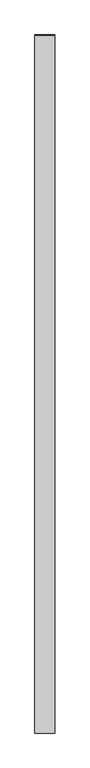
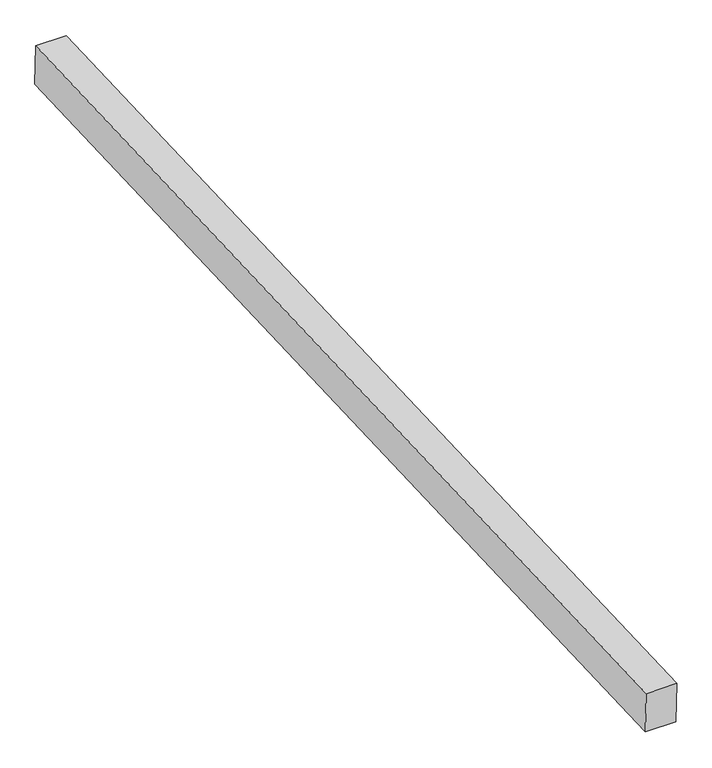
"""IFC4 building model written with IfcOpenShell, lengths in millimetres: proxy geometry, Generic Models 7:Generic Models 1:8:Generic Models 1:8 : Generic Models 7:Generic Models 1:337419:53 : Generic Models 7:Generic Models 1:8:Generic Models 1:8 : Generic Models 7:Generic Models 1:337419:315935."""

from ifc_helpers import new_model, si_unit, frame, origin, place, context, project, spatial, polyline, outline, extrude, source, transform, mapped, element, save


def generic_models_2183cbec(model_context):
    return source(origin(), model_context, "Body", "SweptSolid", [
        extrude(outline(polyline([(-581229.2495411, 3818.908703), (-576356.3266468, 4021.9471569), (-576348.7597251, 3831.5971524), (-581221.3189223, 3628.5738526), (-581229.2495411, 3818.908703)])), frame((608371.661724, 0.0, 0.0), z_axis=(1.0, 0.0, 0.0), x_axis=(0.0, 1.0, 0.0)), (0.0, 0.0, 1.0), 139.7),
    ])


if __name__ == "__main__":
    model = new_model("IFC4")
    model_context = context("Model", 3, world=origin())
    ifc_project = project(units=[si_unit("LENGTHUNIT", "METRE", prefix="MILLI")], contexts=[model_context])
    site = spatial("IfcSite", under=ifc_project)
    building = spatial("IfcBuilding", under=site)
    placement = place(None, origin())
    generic_models_shape = generic_models_2183cbec(model_context)
    element("IfcBuildingElementProxy", 1, Name="Generic Models 7:Generic Models 1:8:Generic Models 1:8 : Generic Models 7:Generic Models 1:337419:53 : Generic Models 7:Generic Models 1:8:Generic Models 1:8 : Generic Models 7:Generic Models 1:337419:315935", ObjectType="Generic Models 7:Generic Models 1:8:Generic Models 1:8 : Generic Models 7:Generic Models 1:337419:53 : Generic Models 7:Generic Models 1:8:Generic Models 1:8 : Generic Models 7:Generic Models 1:337419:315935", at=placement, inside=building, context=model_context, shape_type="MappedRepresentation", body=[
        mapped(generic_models_shape, transform((0.0, 0.0, 0.0), x_axis=(1.0, 0.0, 0.0), y_axis=(0.0, 1.0, 0.0), z_axis=(0.0, 0.0, 1.0))),
    ])
    save(model, "model.ifc")

# Revit data of these elements
# Type "Generic Models 7:Generic Models 1:8:Generic Models 1:8 : Generic Models 7:Generic Models 1:337419:53 : Generic Models 7:Generic Models 1:8:Generic Models 1:8 : Generic Models 7:Generic Models 1:337419:315935"
#   NameOverride = "Generic Models 7:Generic Models 1:8:Generic Models 1:8 : Generic Models 7:Generic Models 1:337419:315935"
#   ObjectTypeOverride = "Generic Models 1:8 : Generic Models 7:Generic Models 1:337419"
#   Reference = "Generic Models 1"
#   Tag = "315935"
# Element 1 (IfcBuildingElementProxy, "Generic Models 7:Generic Models 1:8:Generic Models 1:8 : Generic Models 7:Generic Models 1:337419:53 : Generic Models 7:Generic Models 1:8:Generic Models 1:8 : Generic Models 7:Generic Models 1:337419:315935")
#   Materials on its faces: "5 1/2\" X 7 1/2\" EXTERIOR GRADE GLULAM BEAMS"
# Materials
#   "5 1/2\" X 7 1/2\" EXTERIOR GRADE GLULAM BEAMS": class "Wood", colour RGB 183 134 68, transparency 0, Keynote = "M06181300.01", Description = "Pinus Echinata", Cost = 0
